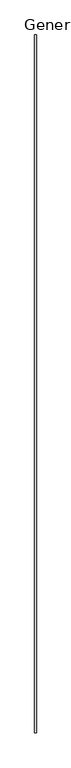
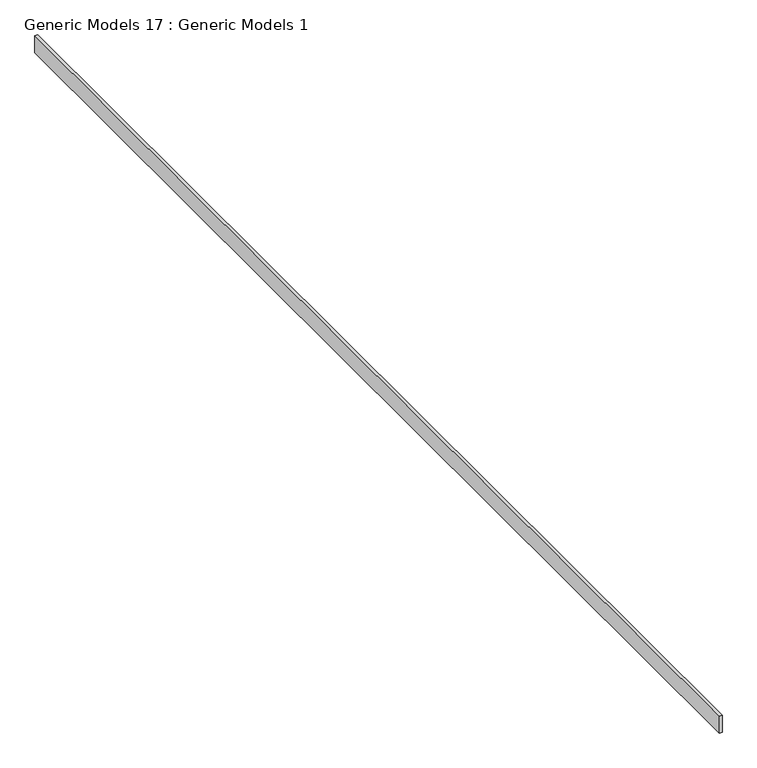
"""IFC4 building model written with IfcOpenShell, lengths in millimetres: proxy geometry, Generic Models 17 : Generic Models 1."""

from ifc_helpers import new_model, si_unit, frame, origin, place, context, project, spatial, polyline, outline, extrude, source, transform, mapped, element, save


def generic_models_17_generic_models_1_9f279b2d(model_context):
    return source(origin(), model_context, "Body", "SweptSolid", [
        extrude(outline(polyline([(8531.0513705, 11981.8769662), (8575.5013705, 11981.8769662), (8575.5013705, -7068.1230338), (8531.0513705, -7068.1230338), (8531.0513705, 11981.8769662)])), frame((0.0, 0.0, 126485.396), z_axis=(0.0, 0.0, 1.0), x_axis=(1.0, 0.0, 0.0)), (0.0, 0.0, 1.0), 285.75),
    ])


if __name__ == "__main__":
    model = new_model("IFC4")
    model_context = context("Model", 3, world=origin())
    ifc_project = project(units=[si_unit("LENGTHUNIT", "METRE", prefix="MILLI")], contexts=[model_context])
    site = spatial("IfcSite", under=ifc_project)
    building = spatial("IfcBuilding", under=site)
    placement = place(None, origin())
    generic_models_17_generic_models_1_shape = generic_models_17_generic_models_1_9f279b2d(model_context)
    element("IfcBuildingElementProxy", 1, Name="Generic Models 17 : Generic Models 1", ObjectType="Generic Models 17 : Generic Models 1", at=placement, inside=building, context=model_context, shape_type="MappedRepresentation", body=[
        mapped(generic_models_17_generic_models_1_shape, transform((0.0, 0.0, 0.0), x_axis=(1.0, 0.0, 0.0), y_axis=(0.0, 1.0, 0.0), z_axis=(0.0, 0.0, 1.0))),
    ])
    save(model, "model.ifc")

# Revit data of these elements
# Element 1 (IfcBuildingElementProxy, "Generic Models 17 : Generic Models 1")
#   Materials on its faces: "_STRUCTURAL MEMBER (SEE STRUCT. DWGS)"
# Materials
#   "_STRUCTURAL MEMBER (SEE STRUCT. DWGS)": class "Generic", colour RGB 209 182 141, transparency 0, Cost = 0
